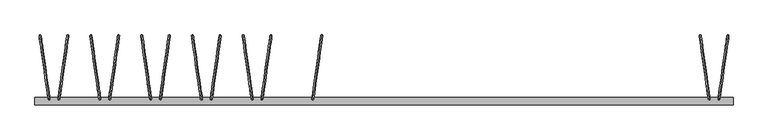
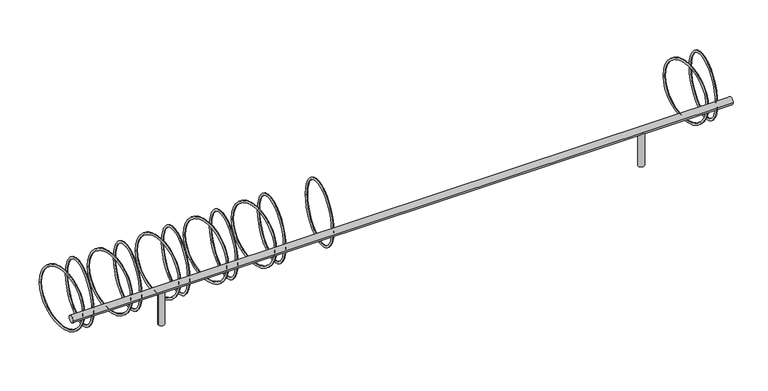
"""IFC4 building model written with IfcOpenShell, lengths in millimetres: geographic element geometry, NLRS_90_SI_WPB_fietsenrek staal_gen_bf : fietsenrek 5500mm 14 plaatsen."""

from ifc_helpers import new_model, si_unit, point, frame, frame_2d, origin, origin_with_axes, place, context, project, spatial, circle_curve, ellipse_curve, trimmed, segment, composite_curve, outline, extrude, source, transform, mapped, element, save
from ifc_brep_helpers import revolved_surface, advanced_brep


def geographic_element_aea35ce9(model_context):
    return source(origin(), model_context, "Body", "SolidModel", [
        advanced_brep(
        [(-560.5888305, 21.9255981, 304.7993564), (-562.7982034, 6.2050925, 304.7993564), (-489.8888952, 524.981777, 304.7993564), (-492.0982681, 509.2612714, 304.7993564)],
        [
            (0, 1, circle_curve(frame((-561.6935169, 14.0653453, 304.7993564), z_axis=(0.0, 0.0, 1.0), x_axis=(0.13917310096005764, 0.9902680687415715, 0.0)), 7.9375)),
            (1, 2, circle_curve(frame((-526.3435493, 265.5934347, 304.7993564), z_axis=(-0.9902680687415715, 0.1391731009600577, 0.0), x_axis=(0.1391731009600577, 0.9902680687415715, 0.0)), 261.9375)),
            (2, 3, circle_curve(frame((-490.9935817, 517.1215242, 304.7993564), z_axis=(0.0, 0.0, 1.0), x_axis=(-0.13917310096005775, -0.9902680687415715, 0.0)), 7.9375)),
            (3, 0, circle_curve(frame((-526.3435493, 265.5934347, 304.7993564), z_axis=(0.9902680687415715, -0.1391731009600577, 0.0), x_axis=(0.1391731009600577, 0.9902680687415715, 0.0)), 246.0625)),
            (1, 0, circle_curve(frame((-561.6935169, 14.0653453, 304.7993564), z_axis=(0.0, 0.0, 1.0), x_axis=(0.13917310096005764, 0.9902680687415715, 0.0)), 7.9375)),
            (3, 2, circle_curve(frame((-490.9935817, 517.1215242, 304.7993564), z_axis=(0.0, 0.0, 1.0), x_axis=(-0.13917310096005775, -0.9902680687415715, 0.0)), 7.9375)),
            (2, 1, circle_curve(frame((-526.3435493, 265.5934347, 304.7993564), z_axis=(-0.9902680687415715, 0.1391731009600577, 0.0), x_axis=(-0.1391731009600577, -0.9902680687415715, 0.0)), 261.9375)),
            (0, 3, circle_curve(frame((-526.3435493, 265.5934347, 304.7993564), z_axis=(0.9902680687415715, -0.1391731009600577, 0.0), x_axis=(-0.1391731009600577, -0.9902680687415715, 0.0)), 246.0625)),
        ],
        [
            revolved_surface(trimmed(ellipse_curve(frame((-490.9935817, 517.1215242, 304.7993564), z_axis=(0.0, 0.0, 1.0), x_axis=(-0.13917310096005775, -0.9902680687415715, 0.0)), 7.9375, 7.9375), [point((-489.8888952, 524.981777, 304.7993564))], [point((-492.0982681, 509.2612714, 304.7993564))], True, "CARTESIAN"), (-714.9896164, 292.1059105, 304.7993564), (-0.9902680687415715, 0.1391731009600577, 0.0)),
            revolved_surface(trimmed(ellipse_curve(frame((-490.9935817, 517.1215242, 304.7993564), z_axis=(0.0, 0.0, 1.0), x_axis=(-0.13917310096005775, -0.9902680687415715, 0.0)), 7.9375, 7.9375), [point((-492.0982681, 509.2612714, 304.7993564))], [point((-489.8888952, 524.981777, 304.7993564))], True, "CARTESIAN"), (-714.9896164, 292.1059105, 304.7993564), (-0.9902680687415715, 0.1391731009600577, 0.0)),
            revolved_surface(trimmed(ellipse_curve(frame((-561.6935169, 14.0653453, 304.7993564), z_axis=(0.0, 0.0, -1.0), x_axis=(0.1391731009600577, 0.9902680687415715, 0.0)), 7.9375, 7.9375), [point((-562.7982034, 6.2050925, 304.7993564))], [point((-560.5888305, 21.9255981, 304.7993564))], True, "CARTESIAN"), (-714.9896164, 292.1059105, 304.7993564), (-0.9902680687415715, 0.1391731009600577, 0.0)),
            revolved_surface(trimmed(ellipse_curve(frame((-561.6935169, 14.0653453, 304.7993564), z_axis=(0.0, 0.0, -1.0), x_axis=(0.1391731009600577, 0.9902680687415715, 0.0)), 7.9375, 7.9375), [point((-560.5888305, 21.9255981, 304.7993564))], [point((-562.7982034, 6.2050925, 304.7993564))], True, "CARTESIAN"), (-714.9896164, 292.1059105, 304.7993564), (-0.9902680687415715, 0.1391731009600577, 0.0)),
        ],
        [
            (0, [[1, 2, 3, 4]]),
            (1, [[5, -4, 6, -2]]),
            (2, [[-3, 7, -1, 8]]),
            (3, [[-6, -8, -5, -7]]),
        ],
    ),
        advanced_brep(
        [(-1039.4111695, 21.9255981, 304.7993564), (-1037.2017966, 6.2050925, 304.7993564), (-1110.1111048, 524.981777, 304.7993564), (-1107.9017319, 509.2612714, 304.7993564)],
        [
            (0, 1, circle_curve(frame((-1038.3064831, 14.0653453, 304.7993564), z_axis=(0.0, 0.0, 1.0), x_axis=(-0.1391731009600606, 0.990268068741571, 0.0)), 7.9375)),
            (1, 2, circle_curve(frame((-1073.6564507, 265.5934347, 304.7993564), z_axis=(-0.990268068741571, -0.13917310096006058, 0.0), x_axis=(-0.13917310096006058, 0.990268068741571, 0.0)), 261.9375)),
            (2, 3, circle_curve(frame((-1109.0064183, 517.1215242, 304.7993564), z_axis=(0.0, 0.0, 1.0), x_axis=(0.13917310096006055, -0.990268068741571, 0.0)), 7.9375)),
            (3, 0, circle_curve(frame((-1073.6564507, 265.5934347, 304.7993564), z_axis=(0.990268068741571, 0.13917310096006058, 0.0), x_axis=(-0.13917310096006058, 0.990268068741571, 0.0)), 246.0625)),
            (1, 0, circle_curve(frame((-1038.3064831, 14.0653453, 304.7993564), z_axis=(0.0, 0.0, 1.0), x_axis=(-0.1391731009600606, 0.990268068741571, 0.0)), 7.9375)),
            (3, 2, circle_curve(frame((-1109.0064183, 517.1215242, 304.7993564), z_axis=(0.0, 0.0, 1.0), x_axis=(0.13917310096006055, -0.990268068741571, 0.0)), 7.9375)),
            (2, 1, circle_curve(frame((-1073.6564507, 265.5934347, 304.7993564), z_axis=(-0.990268068741571, -0.13917310096006058, 0.0), x_axis=(0.13917310096006058, -0.990268068741571, 0.0)), 261.9375)),
            (0, 3, circle_curve(frame((-1073.6564507, 265.5934347, 304.7993564), z_axis=(0.990268068741571, 0.13917310096006058, 0.0), x_axis=(0.13917310096006058, -0.990268068741571, 0.0)), 246.0625)),
        ],
        [
            revolved_surface(trimmed(ellipse_curve(frame((-1109.0064183, 517.1215242, 304.7993564), z_axis=(0.0, 0.0, 1.0), x_axis=(0.13917310096006055, -0.990268068741571, 0.0)), 7.9375, 7.9375), [point((-1110.1111048, 524.981777, 304.7993564))], [point((-1107.9017319, 509.2612714, 304.7993564))], True, "CARTESIAN"), (-885.0103836, 292.1059105, 304.7993564), (-0.990268068741571, -0.13917310096006058, 0.0)),
            revolved_surface(trimmed(ellipse_curve(frame((-1109.0064183, 517.1215242, 304.7993564), z_axis=(0.0, 0.0, 1.0), x_axis=(0.13917310096006055, -0.990268068741571, 0.0)), 7.9375, 7.9375), [point((-1107.9017319, 509.2612714, 304.7993564))], [point((-1110.1111048, 524.981777, 304.7993564))], True, "CARTESIAN"), (-885.0103836, 292.1059105, 304.7993564), (-0.990268068741571, -0.13917310096006058, 0.0)),
            revolved_surface(trimmed(ellipse_curve(frame((-1038.3064831, 14.0653453, 304.7993564), z_axis=(0.0, 0.0, -1.0), x_axis=(-0.13917310096006055, 0.990268068741571, 0.0)), 7.9375, 7.9375), [point((-1037.2017966, 6.2050925, 304.7993564))], [point((-1039.4111695, 21.9255981, 304.7993564))], True, "CARTESIAN"), (-885.0103836, 292.1059105, 304.7993564), (-0.990268068741571, -0.13917310096006058, 0.0)),
            revolved_surface(trimmed(ellipse_curve(frame((-1038.3064831, 14.0653453, 304.7993564), z_axis=(0.0, 0.0, -1.0), x_axis=(-0.13917310096006055, 0.990268068741571, 0.0)), 7.9375, 7.9375), [point((-1039.4111695, 21.9255981, 304.7993564))], [point((-1037.2017966, 6.2050925, 304.7993564))], True, "CARTESIAN"), (-885.0103836, 292.1059105, 304.7993564), (-0.990268068741571, -0.13917310096006058, 0.0)),
        ],
        [
            (0, [[1, 2, 3, 4]]),
            (1, [[5, -4, 6, -2]]),
            (2, [[-3, 7, -1, 8]]),
            (3, [[-6, -8, -5, -7]]),
        ],
    ),
        advanced_brep(
        [(-960.5888305, 21.9255981, 304.7993564), (-962.7982034, 6.2050925, 304.7993564), (-889.8888952, 524.981777, 304.7993564), (-892.0982681, 509.2612714, 304.7993564)],
        [
            (0, 1, circle_curve(frame((-961.6935169, 14.0653453, 304.7993564), z_axis=(0.0, 0.0, 1.0), x_axis=(0.13917310096005764, 0.9902680687415715, 0.0)), 7.9375)),
            (1, 2, circle_curve(frame((-926.3435493, 265.5934347, 304.7993564), z_axis=(-0.9902680687415715, 0.1391731009600577, 0.0), x_axis=(0.1391731009600577, 0.9902680687415715, 0.0)), 261.9375)),
            (2, 3, circle_curve(frame((-890.9935817, 517.1215242, 304.7993564), z_axis=(0.0, 0.0, 1.0), x_axis=(-0.13917310096005775, -0.9902680687415715, 0.0)), 7.9375)),
            (3, 0, circle_curve(frame((-926.3435493, 265.5934347, 304.7993564), z_axis=(0.9902680687415715, -0.1391731009600577, 0.0), x_axis=(0.1391731009600577, 0.9902680687415715, 0.0)), 246.0625)),
            (1, 0, circle_curve(frame((-961.6935169, 14.0653453, 304.7993564), z_axis=(0.0, 0.0, 1.0), x_axis=(0.13917310096005764, 0.9902680687415715, 0.0)), 7.9375)),
            (3, 2, circle_curve(frame((-890.9935817, 517.1215242, 304.7993564), z_axis=(0.0, 0.0, 1.0), x_axis=(-0.13917310096005775, -0.9902680687415715, 0.0)), 7.9375)),
            (2, 1, circle_curve(frame((-926.3435493, 265.5934347, 304.7993564), z_axis=(-0.9902680687415715, 0.1391731009600577, 0.0), x_axis=(-0.1391731009600577, -0.9902680687415715, 0.0)), 261.9375)),
            (0, 3, circle_curve(frame((-926.3435493, 265.5934347, 304.7993564), z_axis=(0.9902680687415715, -0.1391731009600577, 0.0), x_axis=(-0.1391731009600577, -0.9902680687415715, 0.0)), 246.0625)),
        ],
        [
            revolved_surface(trimmed(ellipse_curve(frame((-890.9935817, 517.1215242, 304.7993564), z_axis=(0.0, 0.0, 1.0), x_axis=(-0.13917310096005775, -0.9902680687415715, 0.0)), 7.9375, 7.9375), [point((-889.8888952, 524.981777, 304.7993564))], [point((-892.0982681, 509.2612714, 304.7993564))], True, "CARTESIAN"), (-1114.9896164, 292.1059105, 304.7993564), (-0.9902680687415715, 0.1391731009600577, 0.0)),
            revolved_surface(trimmed(ellipse_curve(frame((-890.9935817, 517.1215242, 304.7993564), z_axis=(0.0, 0.0, 1.0), x_axis=(-0.13917310096005775, -0.9902680687415715, 0.0)), 7.9375, 7.9375), [point((-892.0982681, 509.2612714, 304.7993564))], [point((-889.8888952, 524.981777, 304.7993564))], True, "CARTESIAN"), (-1114.9896164, 292.1059105, 304.7993564), (-0.9902680687415715, 0.1391731009600577, 0.0)),
            revolved_surface(trimmed(ellipse_curve(frame((-961.6935169, 14.0653453, 304.7993564), z_axis=(0.0, 0.0, -1.0), x_axis=(0.1391731009600577, 0.9902680687415715, 0.0)), 7.9375, 7.9375), [point((-962.7982034, 6.2050925, 304.7993564))], [point((-960.5888305, 21.9255981, 304.7993564))], True, "CARTESIAN"), (-1114.9896164, 292.1059105, 304.7993564), (-0.9902680687415715, 0.1391731009600577, 0.0)),
            revolved_surface(trimmed(ellipse_curve(frame((-961.6935169, 14.0653453, 304.7993564), z_axis=(0.0, 0.0, -1.0), x_axis=(0.1391731009600577, 0.9902680687415715, 0.0)), 7.9375, 7.9375), [point((-960.5888305, 21.9255981, 304.7993564))], [point((-962.7982034, 6.2050925, 304.7993564))], True, "CARTESIAN"), (-1114.9896164, 292.1059105, 304.7993564), (-0.9902680687415715, 0.1391731009600577, 0.0)),
        ],
        [
            (0, [[1, 2, 3, 4]]),
            (1, [[5, -4, 6, -2]]),
            (2, [[-3, 7, -1, 8]]),
            (3, [[-6, -8, -5, -7]]),
        ],
    ),
        advanced_brep(
        [(-1439.4111695, 21.9255981, 304.7993564), (-1437.2017966, 6.2050925, 304.7993564), (-1510.1111048, 524.981777, 304.7993564), (-1507.9017319, 509.2612714, 304.7993564)],
        [
            (0, 1, circle_curve(frame((-1438.3064831, 14.0653453, 304.7993564), z_axis=(0.0, 0.0, 1.0), x_axis=(-0.1391731009600606, 0.990268068741571, 0.0)), 7.9375)),
            (1, 2, circle_curve(frame((-1473.6564507, 265.5934347, 304.7993564), z_axis=(-0.990268068741571, -0.13917310096006058, 0.0), x_axis=(-0.13917310096006058, 0.990268068741571, 0.0)), 261.9375)),
            (2, 3, circle_curve(frame((-1509.0064183, 517.1215242, 304.7993564), z_axis=(0.0, 0.0, 1.0), x_axis=(0.13917310096006055, -0.990268068741571, 0.0)), 7.9375)),
            (3, 0, circle_curve(frame((-1473.6564507, 265.5934347, 304.7993564), z_axis=(0.990268068741571, 0.13917310096006058, 0.0), x_axis=(-0.13917310096006058, 0.990268068741571, 0.0)), 246.0625)),
            (1, 0, circle_curve(frame((-1438.3064831, 14.0653453, 304.7993564), z_axis=(0.0, 0.0, 1.0), x_axis=(-0.1391731009600606, 0.990268068741571, 0.0)), 7.9375)),
            (3, 2, circle_curve(frame((-1509.0064183, 517.1215242, 304.7993564), z_axis=(0.0, 0.0, 1.0), x_axis=(0.13917310096006055, -0.990268068741571, 0.0)), 7.9375)),
            (2, 1, circle_curve(frame((-1473.6564507, 265.5934347, 304.7993564), z_axis=(-0.990268068741571, -0.13917310096006058, 0.0), x_axis=(0.13917310096006058, -0.990268068741571, 0.0)), 261.9375)),
            (0, 3, circle_curve(frame((-1473.6564507, 265.5934347, 304.7993564), z_axis=(0.990268068741571, 0.13917310096006058, 0.0), x_axis=(0.13917310096006058, -0.990268068741571, 0.0)), 246.0625)),
        ],
        [
            revolved_surface(trimmed(ellipse_curve(frame((-1509.0064183, 517.1215242, 304.7993564), z_axis=(0.0, 0.0, 1.0), x_axis=(0.13917310096006055, -0.990268068741571, 0.0)), 7.9375, 7.9375), [point((-1510.1111048, 524.981777, 304.7993564))], [point((-1507.9017319, 509.2612714, 304.7993564))], True, "CARTESIAN"), (-1285.0103836, 292.1059105, 304.7993564), (-0.990268068741571, -0.13917310096006058, 0.0)),
            revolved_surface(trimmed(ellipse_curve(frame((-1509.0064183, 517.1215242, 304.7993564), z_axis=(0.0, 0.0, 1.0), x_axis=(0.13917310096006055, -0.990268068741571, 0.0)), 7.9375, 7.9375), [point((-1507.9017319, 509.2612714, 304.7993564))], [point((-1510.1111048, 524.981777, 304.7993564))], True, "CARTESIAN"), (-1285.0103836, 292.1059105, 304.7993564), (-0.990268068741571, -0.13917310096006058, 0.0)),
            revolved_surface(trimmed(ellipse_curve(frame((-1438.3064831, 14.0653453, 304.7993564), z_axis=(0.0, 0.0, -1.0), x_axis=(-0.13917310096006055, 0.990268068741571, 0.0)), 7.9375, 7.9375), [point((-1437.2017966, 6.2050925, 304.7993564))], [point((-1439.4111695, 21.9255981, 304.7993564))], True, "CARTESIAN"), (-1285.0103836, 292.1059105, 304.7993564), (-0.990268068741571, -0.13917310096006058, 0.0)),
            revolved_surface(trimmed(ellipse_curve(frame((-1438.3064831, 14.0653453, 304.7993564), z_axis=(0.0, 0.0, -1.0), x_axis=(-0.13917310096006055, 0.990268068741571, 0.0)), 7.9375, 7.9375), [point((-1439.4111695, 21.9255981, 304.7993564))], [point((-1437.2017966, 6.2050925, 304.7993564))], True, "CARTESIAN"), (-1285.0103836, 292.1059105, 304.7993564), (-0.990268068741571, -0.13917310096006058, 0.0)),
        ],
        [
            (0, [[1, 2, 3, 4]]),
            (1, [[5, -4, 6, -2]]),
            (2, [[-3, 7, -1, 8]]),
            (3, [[-6, -8, -5, -7]]),
        ],
    ),
        advanced_brep(
        [(-1360.5888305, 21.9255981, 304.7993564), (-1362.7982034, 6.2050925, 304.7993564), (-1289.8888952, 524.981777, 304.7993564), (-1292.0982681, 509.2612714, 304.7993564)],
        [
            (0, 1, circle_curve(frame((-1361.6935169, 14.0653453, 304.7993564), z_axis=(0.0, 0.0, 1.0), x_axis=(0.13917310096005764, 0.9902680687415715, 0.0)), 7.9375)),
            (1, 2, circle_curve(frame((-1326.3435493, 265.5934347, 304.7993564), z_axis=(-0.9902680687415715, 0.1391731009600577, 0.0), x_axis=(0.1391731009600577, 0.9902680687415715, 0.0)), 261.9375)),
            (2, 3, circle_curve(frame((-1290.9935817, 517.1215242, 304.7993564), z_axis=(0.0, 0.0, 1.0), x_axis=(-0.13917310096005775, -0.9902680687415715, 0.0)), 7.9375)),
            (3, 0, circle_curve(frame((-1326.3435493, 265.5934347, 304.7993564), z_axis=(0.9902680687415715, -0.1391731009600577, 0.0), x_axis=(0.1391731009600577, 0.9902680687415715, 0.0)), 246.0625)),
            (1, 0, circle_curve(frame((-1361.6935169, 14.0653453, 304.7993564), z_axis=(0.0, 0.0, 1.0), x_axis=(0.13917310096005764, 0.9902680687415715, 0.0)), 7.9375)),
            (3, 2, circle_curve(frame((-1290.9935817, 517.1215242, 304.7993564), z_axis=(0.0, 0.0, 1.0), x_axis=(-0.13917310096005775, -0.9902680687415715, 0.0)), 7.9375)),
            (2, 1, circle_curve(frame((-1326.3435493, 265.5934347, 304.7993564), z_axis=(-0.9902680687415715, 0.1391731009600577, 0.0), x_axis=(-0.1391731009600577, -0.9902680687415715, 0.0)), 261.9375)),
            (0, 3, circle_curve(frame((-1326.3435493, 265.5934347, 304.7993564), z_axis=(0.9902680687415715, -0.1391731009600577, 0.0), x_axis=(-0.1391731009600577, -0.9902680687415715, 0.0)), 246.0625)),
        ],
        [
            revolved_surface(trimmed(ellipse_curve(frame((-1290.9935817, 517.1215242, 304.7993564), z_axis=(0.0, 0.0, 1.0), x_axis=(-0.13917310096005775, -0.9902680687415715, 0.0)), 7.9375, 7.9375), [point((-1289.8888952, 524.981777, 304.7993564))], [point((-1292.0982681, 509.2612714, 304.7993564))], True, "CARTESIAN"), (-1514.9896164, 292.1059105, 304.7993564), (-0.9902680687415715, 0.1391731009600577, 0.0)),
            revolved_surface(trimmed(ellipse_curve(frame((-1290.9935817, 517.1215242, 304.7993564), z_axis=(0.0, 0.0, 1.0), x_axis=(-0.13917310096005775, -0.9902680687415715, 0.0)), 7.9375, 7.9375), [point((-1292.0982681, 509.2612714, 304.7993564))], [point((-1289.8888952, 524.981777, 304.7993564))], True, "CARTESIAN"), (-1514.9896164, 292.1059105, 304.7993564), (-0.9902680687415715, 0.1391731009600577, 0.0)),
            revolved_surface(trimmed(ellipse_curve(frame((-1361.6935169, 14.0653453, 304.7993564), z_axis=(0.0, 0.0, -1.0), x_axis=(0.1391731009600577, 0.9902680687415715, 0.0)), 7.9375, 7.9375), [point((-1362.7982034, 6.2050925, 304.7993564))], [point((-1360.5888305, 21.9255981, 304.7993564))], True, "CARTESIAN"), (-1514.9896164, 292.1059105, 304.7993564), (-0.9902680687415715, 0.1391731009600577, 0.0)),
            revolved_surface(trimmed(ellipse_curve(frame((-1361.6935169, 14.0653453, 304.7993564), z_axis=(0.0, 0.0, -1.0), x_axis=(0.1391731009600577, 0.9902680687415715, 0.0)), 7.9375, 7.9375), [point((-1360.5888305, 21.9255981, 304.7993564))], [point((-1362.7982034, 6.2050925, 304.7993564))], True, "CARTESIAN"), (-1514.9896164, 292.1059105, 304.7993564), (-0.9902680687415715, 0.1391731009600577, 0.0)),
        ],
        [
            (0, [[1, 2, 3, 4]]),
            (1, [[5, -4, 6, -2]]),
            (2, [[-3, 7, -1, 8]]),
            (3, [[-6, -8, -5, -7]]),
        ],
    ),
        advanced_brep(
        [(-1839.4111695, 21.9255981, 304.7993564), (-1837.2017966, 6.2050925, 304.7993564), (-1910.1111048, 524.981777, 304.7993564), (-1907.9017319, 509.2612714, 304.7993564)],
        [
            (0, 1, circle_curve(frame((-1838.3064831, 14.0653453, 304.7993564), z_axis=(0.0, 0.0, 1.0), x_axis=(-0.1391731009600606, 0.990268068741571, 0.0)), 7.9375)),
            (1, 2, circle_curve(frame((-1873.6564507, 265.5934347, 304.7993564), z_axis=(-0.990268068741571, -0.13917310096006058, 0.0), x_axis=(-0.13917310096006058, 0.990268068741571, 0.0)), 261.9375)),
            (2, 3, circle_curve(frame((-1909.0064183, 517.1215242, 304.7993564), z_axis=(0.0, 0.0, 1.0), x_axis=(0.13917310096006055, -0.990268068741571, 0.0)), 7.9375)),
            (3, 0, circle_curve(frame((-1873.6564507, 265.5934347, 304.7993564), z_axis=(0.990268068741571, 0.13917310096006058, 0.0), x_axis=(-0.13917310096006058, 0.990268068741571, 0.0)), 246.0625)),
            (1, 0, circle_curve(frame((-1838.3064831, 14.0653453, 304.7993564), z_axis=(0.0, 0.0, 1.0), x_axis=(-0.1391731009600606, 0.990268068741571, 0.0)), 7.9375)),
            (3, 2, circle_curve(frame((-1909.0064183, 517.1215242, 304.7993564), z_axis=(0.0, 0.0, 1.0), x_axis=(0.13917310096006055, -0.990268068741571, 0.0)), 7.9375)),
            (2, 1, circle_curve(frame((-1873.6564507, 265.5934347, 304.7993564), z_axis=(-0.990268068741571, -0.13917310096006058, 0.0), x_axis=(0.13917310096006058, -0.990268068741571, 0.0)), 261.9375)),
            (0, 3, circle_curve(frame((-1873.6564507, 265.5934347, 304.7993564), z_axis=(0.990268068741571, 0.13917310096006058, 0.0), x_axis=(0.13917310096006058, -0.990268068741571, 0.0)), 246.0625)),
        ],
        [
            revolved_surface(trimmed(ellipse_curve(frame((-1909.0064183, 517.1215242, 304.7993564), z_axis=(0.0, 0.0, 1.0), x_axis=(0.13917310096006055, -0.990268068741571, 0.0)), 7.9375, 7.9375), [point((-1910.1111048, 524.981777, 304.7993564))], [point((-1907.9017319, 509.2612714, 304.7993564))], True, "CARTESIAN"), (-1685.0103836, 292.1059105, 304.7993564), (-0.990268068741571, -0.13917310096006058, 0.0)),
            revolved_surface(trimmed(ellipse_curve(frame((-1909.0064183, 517.1215242, 304.7993564), z_axis=(0.0, 0.0, 1.0), x_axis=(0.13917310096006055, -0.990268068741571, 0.0)), 7.9375, 7.9375), [point((-1907.9017319, 509.2612714, 304.7993564))], [point((-1910.1111048, 524.981777, 304.7993564))], True, "CARTESIAN"), (-1685.0103836, 292.1059105, 304.7993564), (-0.990268068741571, -0.13917310096006058, 0.0)),
            revolved_surface(trimmed(ellipse_curve(frame((-1838.3064831, 14.0653453, 304.7993564), z_axis=(0.0, 0.0, -1.0), x_axis=(-0.13917310096006055, 0.990268068741571, 0.0)), 7.9375, 7.9375), [point((-1837.2017966, 6.2050925, 304.7993564))], [point((-1839.4111695, 21.9255981, 304.7993564))], True, "CARTESIAN"), (-1685.0103836, 292.1059105, 304.7993564), (-0.990268068741571, -0.13917310096006058, 0.0)),
            revolved_surface(trimmed(ellipse_curve(frame((-1838.3064831, 14.0653453, 304.7993564), z_axis=(0.0, 0.0, -1.0), x_axis=(-0.13917310096006055, 0.990268068741571, 0.0)), 7.9375, 7.9375), [point((-1839.4111695, 21.9255981, 304.7993564))], [point((-1837.2017966, 6.2050925, 304.7993564))], True, "CARTESIAN"), (-1685.0103836, 292.1059105, 304.7993564), (-0.990268068741571, -0.13917310096006058, 0.0)),
        ],
        [
            (0, [[1, 2, 3, 4]]),
            (1, [[5, -4, 6, -2]]),
            (2, [[-3, 7, -1, 8]]),
            (3, [[-6, -8, -5, -7]]),
        ],
    ),
        advanced_brep(
        [(-1760.5888305, 21.9255981, 304.7993564), (-1762.7982034, 6.2050925, 304.7993564), (-1689.8888952, 524.981777, 304.7993564), (-1692.0982681, 509.2612714, 304.7993564)],
        [
            (0, 1, circle_curve(frame((-1761.6935169, 14.0653453, 304.7993564), z_axis=(0.0, 0.0, 1.0), x_axis=(0.13917310096005764, 0.9902680687415715, 0.0)), 7.9375)),
            (1, 2, circle_curve(frame((-1726.3435493, 265.5934347, 304.7993564), z_axis=(-0.9902680687415715, 0.1391731009600577, 0.0), x_axis=(0.1391731009600577, 0.9902680687415715, 0.0)), 261.9375)),
            (2, 3, circle_curve(frame((-1690.9935817, 517.1215242, 304.7993564), z_axis=(0.0, 0.0, 1.0), x_axis=(-0.13917310096005775, -0.9902680687415715, 0.0)), 7.9375)),
            (3, 0, circle_curve(frame((-1726.3435493, 265.5934347, 304.7993564), z_axis=(0.9902680687415715, -0.1391731009600577, 0.0), x_axis=(0.1391731009600577, 0.9902680687415715, 0.0)), 246.0625)),
            (1, 0, circle_curve(frame((-1761.6935169, 14.0653453, 304.7993564), z_axis=(0.0, 0.0, 1.0), x_axis=(0.13917310096005764, 0.9902680687415715, 0.0)), 7.9375)),
            (3, 2, circle_curve(frame((-1690.9935817, 517.1215242, 304.7993564), z_axis=(0.0, 0.0, 1.0), x_axis=(-0.13917310096005775, -0.9902680687415715, 0.0)), 7.9375)),
            (2, 1, circle_curve(frame((-1726.3435493, 265.5934347, 304.7993564), z_axis=(-0.9902680687415715, 0.1391731009600577, 0.0), x_axis=(-0.1391731009600577, -0.9902680687415715, 0.0)), 261.9375)),
            (0, 3, circle_curve(frame((-1726.3435493, 265.5934347, 304.7993564), z_axis=(0.9902680687415715, -0.1391731009600577, 0.0), x_axis=(-0.1391731009600577, -0.9902680687415715, 0.0)), 246.0625)),
        ],
        [
            revolved_surface(trimmed(ellipse_curve(frame((-1690.9935817, 517.1215242, 304.7993564), z_axis=(0.0, 0.0, 1.0), x_axis=(-0.13917310096005775, -0.9902680687415715, 0.0)), 7.9375, 7.9375), [point((-1689.8888952, 524.981777, 304.7993564))], [point((-1692.0982681, 509.2612714, 304.7993564))], True, "CARTESIAN"), (-1914.9896164, 292.1059105, 304.7993564), (-0.9902680687415715, 0.1391731009600577, 0.0)),
            revolved_surface(trimmed(ellipse_curve(frame((-1690.9935817, 517.1215242, 304.7993564), z_axis=(0.0, 0.0, 1.0), x_axis=(-0.13917310096005775, -0.9902680687415715, 0.0)), 7.9375, 7.9375), [point((-1692.0982681, 509.2612714, 304.7993564))], [point((-1689.8888952, 524.981777, 304.7993564))], True, "CARTESIAN"), (-1914.9896164, 292.1059105, 304.7993564), (-0.9902680687415715, 0.1391731009600577, 0.0)),
            revolved_surface(trimmed(ellipse_curve(frame((-1761.6935169, 14.0653453, 304.7993564), z_axis=(0.0, 0.0, -1.0), x_axis=(0.1391731009600577, 0.9902680687415715, 0.0)), 7.9375, 7.9375), [point((-1762.7982034, 6.2050925, 304.7993564))], [point((-1760.5888305, 21.9255981, 304.7993564))], True, "CARTESIAN"), (-1914.9896164, 292.1059105, 304.7993564), (-0.9902680687415715, 0.1391731009600577, 0.0)),
            revolved_surface(trimmed(ellipse_curve(frame((-1761.6935169, 14.0653453, 304.7993564), z_axis=(0.0, 0.0, -1.0), x_axis=(0.1391731009600577, 0.9902680687415715, 0.0)), 7.9375, 7.9375), [point((-1760.5888305, 21.9255981, 304.7993564))], [point((-1762.7982034, 6.2050925, 304.7993564))], True, "CARTESIAN"), (-1914.9896164, 292.1059105, 304.7993564), (-0.9902680687415715, 0.1391731009600577, 0.0)),
        ],
        [
            (0, [[1, 2, 3, 4]]),
            (1, [[5, -4, 6, -2]]),
            (2, [[-3, 7, -1, 8]]),
            (3, [[-6, -8, -5, -7]]),
        ],
    ),
        advanced_brep(
        [(-2239.4111695, 21.9255981, 304.7993564), (-2237.2017966, 6.2050925, 304.7993564), (-2310.1111048, 524.981777, 304.7993564), (-2307.9017319, 509.2612714, 304.7993564)],
        [
            (0, 1, circle_curve(frame((-2238.3064831, 14.0653453, 304.7993564), z_axis=(0.0, 0.0, 1.0), x_axis=(-0.1391731009600606, 0.990268068741571, 0.0)), 7.9375)),
            (1, 2, circle_curve(frame((-2273.6564507, 265.5934347, 304.7993564), z_axis=(-0.990268068741571, -0.13917310096006058, 0.0), x_axis=(-0.13917310096006058, 0.990268068741571, 0.0)), 261.9375)),
            (2, 3, circle_curve(frame((-2309.0064183, 517.1215242, 304.7993564), z_axis=(0.0, 0.0, 1.0), x_axis=(0.13917310096006055, -0.990268068741571, 0.0)), 7.9375)),
            (3, 0, circle_curve(frame((-2273.6564507, 265.5934347, 304.7993564), z_axis=(0.990268068741571, 0.13917310096006058, 0.0), x_axis=(-0.13917310096006058, 0.990268068741571, 0.0)), 246.0625)),
            (1, 0, circle_curve(frame((-2238.3064831, 14.0653453, 304.7993564), z_axis=(0.0, 0.0, 1.0), x_axis=(-0.1391731009600606, 0.990268068741571, 0.0)), 7.9375)),
            (3, 2, circle_curve(frame((-2309.0064183, 517.1215242, 304.7993564), z_axis=(0.0, 0.0, 1.0), x_axis=(0.13917310096006055, -0.990268068741571, 0.0)), 7.9375)),
            (2, 1, circle_curve(frame((-2273.6564507, 265.5934347, 304.7993564), z_axis=(-0.990268068741571, -0.13917310096006058, 0.0), x_axis=(0.13917310096006058, -0.990268068741571, 0.0)), 261.9375)),
            (0, 3, circle_curve(frame((-2273.6564507, 265.5934347, 304.7993564), z_axis=(0.990268068741571, 0.13917310096006058, 0.0), x_axis=(0.13917310096006058, -0.990268068741571, 0.0)), 246.0625)),
        ],
        [
            revolved_surface(trimmed(ellipse_curve(frame((-2309.0064183, 517.1215242, 304.7993564), z_axis=(0.0, 0.0, 1.0), x_axis=(0.13917310096006055, -0.990268068741571, 0.0)), 7.9375, 7.9375), [point((-2310.1111048, 524.981777, 304.7993564))], [point((-2307.9017319, 509.2612714, 304.7993564))], True, "CARTESIAN"), (-2085.0103836, 292.1059105, 304.7993564), (-0.990268068741571, -0.13917310096006058, 0.0)),
            revolved_surface(trimmed(ellipse_curve(frame((-2309.0064183, 517.1215242, 304.7993564), z_axis=(0.0, 0.0, 1.0), x_axis=(0.13917310096006055, -0.990268068741571, 0.0)), 7.9375, 7.9375), [point((-2307.9017319, 509.2612714, 304.7993564))], [point((-2310.1111048, 524.981777, 304.7993564))], True, "CARTESIAN"), (-2085.0103836, 292.1059105, 304.7993564), (-0.990268068741571, -0.13917310096006058, 0.0)),
            revolved_surface(trimmed(ellipse_curve(frame((-2238.3064831, 14.0653453, 304.7993564), z_axis=(0.0, 0.0, -1.0), x_axis=(-0.13917310096006055, 0.990268068741571, 0.0)), 7.9375, 7.9375), [point((-2237.2017966, 6.2050925, 304.7993564))], [point((-2239.4111695, 21.9255981, 304.7993564))], True, "CARTESIAN"), (-2085.0103836, 292.1059105, 304.7993564), (-0.990268068741571, -0.13917310096006058, 0.0)),
            revolved_surface(trimmed(ellipse_curve(frame((-2238.3064831, 14.0653453, 304.7993564), z_axis=(0.0, 0.0, -1.0), x_axis=(-0.13917310096006055, 0.990268068741571, 0.0)), 7.9375, 7.9375), [point((-2239.4111695, 21.9255981, 304.7993564))], [point((-2237.2017966, 6.2050925, 304.7993564))], True, "CARTESIAN"), (-2085.0103836, 292.1059105, 304.7993564), (-0.990268068741571, -0.13917310096006058, 0.0)),
        ],
        [
            (0, [[1, 2, 3, 4]]),
            (1, [[5, -4, 6, -2]]),
            (2, [[-3, 7, -1, 8]]),
            (3, [[-6, -8, -5, -7]]),
        ],
    ),
        advanced_brep(
        [(-2160.5888305, 21.9255981, 304.7993564), (-2162.7982034, 6.2050925, 304.7993564), (-2089.8888952, 524.981777, 304.7993564), (-2092.0982681, 509.2612714, 304.7993564)],
        [
            (0, 1, circle_curve(frame((-2161.6935169, 14.0653453, 304.7993564), z_axis=(0.0, 0.0, 1.0), x_axis=(0.13917310096005764, 0.9902680687415715, 0.0)), 7.9375)),
            (1, 2, circle_curve(frame((-2126.3435493, 265.5934347, 304.7993564), z_axis=(-0.9902680687415715, 0.1391731009600577, 0.0), x_axis=(0.1391731009600577, 0.9902680687415715, 0.0)), 261.9375)),
            (2, 3, circle_curve(frame((-2090.9935817, 517.1215242, 304.7993564), z_axis=(0.0, 0.0, 1.0), x_axis=(-0.13917310096005775, -0.9902680687415715, 0.0)), 7.9375)),
            (3, 0, circle_curve(frame((-2126.3435493, 265.5934347, 304.7993564), z_axis=(0.9902680687415715, -0.1391731009600577, 0.0), x_axis=(0.1391731009600577, 0.9902680687415715, 0.0)), 246.0625)),
            (1, 0, circle_curve(frame((-2161.6935169, 14.0653453, 304.7993564), z_axis=(0.0, 0.0, 1.0), x_axis=(0.13917310096005764, 0.9902680687415715, 0.0)), 7.9375)),
            (3, 2, circle_curve(frame((-2090.9935817, 517.1215242, 304.7993564), z_axis=(0.0, 0.0, 1.0), x_axis=(-0.13917310096005775, -0.9902680687415715, 0.0)), 7.9375)),
            (2, 1, circle_curve(frame((-2126.3435493, 265.5934347, 304.7993564), z_axis=(-0.9902680687415715, 0.1391731009600577, 0.0), x_axis=(-0.1391731009600577, -0.9902680687415715, 0.0)), 261.9375)),
            (0, 3, circle_curve(frame((-2126.3435493, 265.5934347, 304.7993564), z_axis=(0.9902680687415715, -0.1391731009600577, 0.0), x_axis=(-0.1391731009600577, -0.9902680687415715, 0.0)), 246.0625)),
        ],
        [
            revolved_surface(trimmed(ellipse_curve(frame((-2090.9935817, 517.1215242, 304.7993564), z_axis=(0.0, 0.0, 1.0), x_axis=(-0.13917310096005775, -0.9902680687415715, 0.0)), 7.9375, 7.9375), [point((-2089.8888952, 524.981777, 304.7993564))], [point((-2092.0982681, 509.2612714, 304.7993564))], True, "CARTESIAN"), (-2314.9896164, 292.1059105, 304.7993564), (-0.9902680687415715, 0.1391731009600577, 0.0)),
            revolved_surface(trimmed(ellipse_curve(frame((-2090.9935817, 517.1215242, 304.7993564), z_axis=(0.0, 0.0, 1.0), x_axis=(-0.13917310096005775, -0.9902680687415715, 0.0)), 7.9375, 7.9375), [point((-2092.0982681, 509.2612714, 304.7993564))], [point((-2089.8888952, 524.981777, 304.7993564))], True, "CARTESIAN"), (-2314.9896164, 292.1059105, 304.7993564), (-0.9902680687415715, 0.1391731009600577, 0.0)),
            revolved_surface(trimmed(ellipse_curve(frame((-2161.6935169, 14.0653453, 304.7993564), z_axis=(0.0, 0.0, -1.0), x_axis=(0.1391731009600577, 0.9902680687415715, 0.0)), 7.9375, 7.9375), [point((-2162.7982034, 6.2050925, 304.7993564))], [point((-2160.5888305, 21.9255981, 304.7993564))], True, "CARTESIAN"), (-2314.9896164, 292.1059105, 304.7993564), (-0.9902680687415715, 0.1391731009600577, 0.0)),
            revolved_surface(trimmed(ellipse_curve(frame((-2161.6935169, 14.0653453, 304.7993564), z_axis=(0.0, 0.0, -1.0), x_axis=(0.1391731009600577, 0.9902680687415715, 0.0)), 7.9375, 7.9375), [point((-2160.5888305, 21.9255981, 304.7993564))], [point((-2162.7982034, 6.2050925, 304.7993564))], True, "CARTESIAN"), (-2314.9896164, 292.1059105, 304.7993564), (-0.9902680687415715, 0.1391731009600577, 0.0)),
        ],
        [
            (0, [[1, 2, 3, 4]]),
            (1, [[5, -4, 6, -2]]),
            (2, [[-3, 7, -1, 8]]),
            (3, [[-6, -8, -5, -7]]),
        ],
    ),
        advanced_brep(
        [(2560.5888305, 21.9255981, 304.7993564), (2562.7982034, 6.2050925, 304.7993564), (2489.8888952, 524.981777, 304.7993564), (2492.0982681, 509.2612714, 304.7993564)],
        [
            (0, 1, circle_curve(frame((2561.6935169, 14.0653453, 304.7993564), z_axis=(0.0, 0.0, 1.0), x_axis=(-0.1391731009600606, 0.990268068741571, 0.0)), 7.9375)),
            (1, 2, circle_curve(frame((2526.3435493, 265.5934347, 304.7993564), z_axis=(-0.990268068741571, -0.13917310096006058, 0.0), x_axis=(-0.13917310096006058, 0.990268068741571, 0.0)), 261.9375)),
            (2, 3, circle_curve(frame((2490.9935817, 517.1215242, 304.7993564), z_axis=(0.0, 0.0, 1.0), x_axis=(0.13917310096006055, -0.990268068741571, 0.0)), 7.9375)),
            (3, 0, circle_curve(frame((2526.3435493, 265.5934347, 304.7993564), z_axis=(0.990268068741571, 0.13917310096006058, 0.0), x_axis=(-0.13917310096006058, 0.990268068741571, 0.0)), 246.0625)),
            (1, 0, circle_curve(frame((2561.6935169, 14.0653453, 304.7993564), z_axis=(0.0, 0.0, 1.0), x_axis=(-0.1391731009600606, 0.990268068741571, 0.0)), 7.9375)),
            (3, 2, circle_curve(frame((2490.9935817, 517.1215242, 304.7993564), z_axis=(0.0, 0.0, 1.0), x_axis=(0.13917310096006055, -0.990268068741571, 0.0)), 7.9375)),
            (2, 1, circle_curve(frame((2526.3435493, 265.5934347, 304.7993564), z_axis=(-0.990268068741571, -0.13917310096006058, 0.0), x_axis=(0.13917310096006058, -0.990268068741571, 0.0)), 261.9375)),
            (0, 3, circle_curve(frame((2526.3435493, 265.5934347, 304.7993564), z_axis=(0.990268068741571, 0.13917310096006058, 0.0), x_axis=(0.13917310096006058, -0.990268068741571, 0.0)), 246.0625)),
        ],
        [
            revolved_surface(trimmed(ellipse_curve(frame((2490.9935817, 517.1215242, 304.7993564), z_axis=(0.0, 0.0, 1.0), x_axis=(0.13917310096006055, -0.990268068741571, 0.0)), 7.9375, 7.9375), [point((2489.8888952, 524.981777, 304.7993564))], [point((2492.0982681, 509.2612714, 304.7993564))], True, "CARTESIAN"), (2714.9896164, 292.1059105, 304.7993564), (-0.990268068741571, -0.13917310096006058, 0.0)),
            revolved_surface(trimmed(ellipse_curve(frame((2490.9935817, 517.1215242, 304.7993564), z_axis=(0.0, 0.0, 1.0), x_axis=(0.13917310096006055, -0.990268068741571, 0.0)), 7.9375, 7.9375), [point((2492.0982681, 509.2612714, 304.7993564))], [point((2489.8888952, 524.981777, 304.7993564))], True, "CARTESIAN"), (2714.9896164, 292.1059105, 304.7993564), (-0.990268068741571, -0.13917310096006058, 0.0)),
            revolved_surface(trimmed(ellipse_curve(frame((2561.6935169, 14.0653453, 304.7993564), z_axis=(0.0, 0.0, -1.0), x_axis=(-0.13917310096006055, 0.990268068741571, 0.0)), 7.9375, 7.9375), [point((2562.7982034, 6.2050925, 304.7993564))], [point((2560.5888305, 21.9255981, 304.7993564))], True, "CARTESIAN"), (2714.9896164, 292.1059105, 304.7993564), (-0.990268068741571, -0.13917310096006058, 0.0)),
            revolved_surface(trimmed(ellipse_curve(frame((2561.6935169, 14.0653453, 304.7993564), z_axis=(0.0, 0.0, -1.0), x_axis=(-0.13917310096006055, 0.990268068741571, 0.0)), 7.9375, 7.9375), [point((2560.5888305, 21.9255981, 304.7993564))], [point((2562.7982034, 6.2050925, 304.7993564))], True, "CARTESIAN"), (2714.9896164, 292.1059105, 304.7993564), (-0.990268068741571, -0.13917310096006058, 0.0)),
        ],
        [
            (0, [[1, 2, 3, 4]]),
            (1, [[5, -4, 6, -2]]),
            (2, [[-3, 7, -1, 8]]),
            (3, [[-6, -8, -5, -7]]),
        ],
    ),
        advanced_brep(
        [(2639.4111695, 21.9255981, 304.7993564), (2637.2017966, 6.2050925, 304.7993564), (2710.1111048, 524.981777, 304.7993564), (2707.9017319, 509.2612714, 304.7993564)],
        [
            (0, 1, circle_curve(frame((2638.3064831, 14.0653453, 304.7993564), z_axis=(0.0, 0.0, 1.0), x_axis=(0.13917310096005764, 0.9902680687415715, 0.0)), 7.9375)),
            (1, 2, circle_curve(frame((2673.6564507, 265.5934347, 304.7993564), z_axis=(-0.9902680687415715, 0.1391731009600577, 0.0), x_axis=(0.1391731009600577, 0.9902680687415715, 0.0)), 261.9375)),
            (2, 3, circle_curve(frame((2709.0064183, 517.1215242, 304.7993564), z_axis=(0.0, 0.0, 1.0), x_axis=(-0.13917310096005775, -0.9902680687415715, 0.0)), 7.9375)),
            (3, 0, circle_curve(frame((2673.6564507, 265.5934347, 304.7993564), z_axis=(0.9902680687415715, -0.1391731009600577, 0.0), x_axis=(0.1391731009600577, 0.9902680687415715, 0.0)), 246.0625)),
            (1, 0, circle_curve(frame((2638.3064831, 14.0653453, 304.7993564), z_axis=(0.0, 0.0, 1.0), x_axis=(0.13917310096005764, 0.9902680687415715, 0.0)), 7.9375)),
            (3, 2, circle_curve(frame((2709.0064183, 517.1215242, 304.7993564), z_axis=(0.0, 0.0, 1.0), x_axis=(-0.13917310096005775, -0.9902680687415715, 0.0)), 7.9375)),
            (2, 1, circle_curve(frame((2673.6564507, 265.5934347, 304.7993564), z_axis=(-0.9902680687415715, 0.1391731009600577, 0.0), x_axis=(-0.1391731009600577, -0.9902680687415715, 0.0)), 261.9375)),
            (0, 3, circle_curve(frame((2673.6564507, 265.5934347, 304.7993564), z_axis=(0.9902680687415715, -0.1391731009600577, 0.0), x_axis=(-0.1391731009600577, -0.9902680687415715, 0.0)), 246.0625)),
        ],
        [
            revolved_surface(trimmed(ellipse_curve(frame((2709.0064183, 517.1215242, 304.7993564), z_axis=(0.0, 0.0, 1.0), x_axis=(-0.13917310096005775, -0.9902680687415715, 0.0)), 7.9375, 7.9375), [point((2710.1111048, 524.981777, 304.7993564))], [point((2707.9017319, 509.2612714, 304.7993564))], True, "CARTESIAN"), (2485.0103836, 292.1059105, 304.7993564), (-0.9902680687415715, 0.1391731009600577, 0.0)),
            revolved_surface(trimmed(ellipse_curve(frame((2709.0064183, 517.1215242, 304.7993564), z_axis=(0.0, 0.0, 1.0), x_axis=(-0.13917310096005775, -0.9902680687415715, 0.0)), 7.9375, 7.9375), [point((2707.9017319, 509.2612714, 304.7993564))], [point((2710.1111048, 524.981777, 304.7993564))], True, "CARTESIAN"), (2485.0103836, 292.1059105, 304.7993564), (-0.9902680687415715, 0.1391731009600577, 0.0)),
            revolved_surface(trimmed(ellipse_curve(frame((2638.3064831, 14.0653453, 304.7993564), z_axis=(0.0, 0.0, -1.0), x_axis=(0.1391731009600577, 0.9902680687415715, 0.0)), 7.9375, 7.9375), [point((2637.2017966, 6.2050925, 304.7993564))], [point((2639.4111695, 21.9255981, 304.7993564))], True, "CARTESIAN"), (2485.0103836, 292.1059105, 304.7993564), (-0.9902680687415715, 0.1391731009600577, 0.0)),
            revolved_surface(trimmed(ellipse_curve(frame((2638.3064831, 14.0653453, 304.7993564), z_axis=(0.0, 0.0, -1.0), x_axis=(0.1391731009600577, 0.9902680687415715, 0.0)), 7.9375, 7.9375), [point((2639.4111695, 21.9255981, 304.7993564))], [point((2637.2017966, 6.2050925, 304.7993564))], True, "CARTESIAN"), (2485.0103836, 292.1059105, 304.7993564), (-0.9902680687415715, 0.1391731009600577, 0.0)),
        ],
        [
            (0, [[1, 2, 3, 4]]),
            (1, [[5, -4, 6, -2]]),
            (2, [[-3, 7, -1, 8]]),
            (3, [[-6, -8, -5, -7]]),
        ],
    ),
        advanced_brep(
        [(-2639.4111695, 21.9255981, 304.7993564), (-2637.2017966, 6.2050925, 304.7993564), (-2710.1111048, 524.981777, 304.7993564), (-2707.9017319, 509.2612714, 304.7993564)],
        [
            (0, 1, circle_curve(frame((-2638.3064831, 14.0653453, 304.7993564), z_axis=(0.0, 0.0, 1.0), x_axis=(-0.1391731009600606, 0.990268068741571, 0.0)), 7.9375)),
            (1, 2, circle_curve(frame((-2673.6564507, 265.5934347, 304.7993564), z_axis=(-0.990268068741571, -0.13917310096006058, 0.0), x_axis=(-0.13917310096006058, 0.990268068741571, 0.0)), 261.9375)),
            (2, 3, circle_curve(frame((-2709.0064183, 517.1215242, 304.7993564), z_axis=(0.0, 0.0, 1.0), x_axis=(0.13917310096006055, -0.990268068741571, 0.0)), 7.9375)),
            (3, 0, circle_curve(frame((-2673.6564507, 265.5934347, 304.7993564), z_axis=(0.990268068741571, 0.13917310096006058, 0.0), x_axis=(-0.13917310096006058, 0.990268068741571, 0.0)), 246.0625)),
            (1, 0, circle_curve(frame((-2638.3064831, 14.0653453, 304.7993564), z_axis=(0.0, 0.0, 1.0), x_axis=(-0.1391731009600606, 0.990268068741571, 0.0)), 7.9375)),
            (3, 2, circle_curve(frame((-2709.0064183, 517.1215242, 304.7993564), z_axis=(0.0, 0.0, 1.0), x_axis=(0.13917310096006055, -0.990268068741571, 0.0)), 7.9375)),
            (2, 1, circle_curve(frame((-2673.6564507, 265.5934347, 304.7993564), z_axis=(-0.990268068741571, -0.13917310096006058, 0.0), x_axis=(0.13917310096006058, -0.990268068741571, 0.0)), 261.9375)),
            (0, 3, circle_curve(frame((-2673.6564507, 265.5934347, 304.7993564), z_axis=(0.990268068741571, 0.13917310096006058, 0.0), x_axis=(0.13917310096006058, -0.990268068741571, 0.0)), 246.0625)),
        ],
        [
            revolved_surface(trimmed(ellipse_curve(frame((-2709.0064183, 517.1215242, 304.7993564), z_axis=(0.0, 0.0, 1.0), x_axis=(0.13917310096006055, -0.990268068741571, 0.0)), 7.9375, 7.9375), [point((-2710.1111048, 524.981777, 304.7993564))], [point((-2707.9017319, 509.2612714, 304.7993564))], True, "CARTESIAN"), (-2485.0103836, 292.1059105, 304.7993564), (-0.990268068741571, -0.13917310096006058, 0.0)),
            revolved_surface(trimmed(ellipse_curve(frame((-2709.0064183, 517.1215242, 304.7993564), z_axis=(0.0, 0.0, 1.0), x_axis=(0.13917310096006055, -0.990268068741571, 0.0)), 7.9375, 7.9375), [point((-2707.9017319, 509.2612714, 304.7993564))], [point((-2710.1111048, 524.981777, 304.7993564))], True, "CARTESIAN"), (-2485.0103836, 292.1059105, 304.7993564), (-0.990268068741571, -0.13917310096006058, 0.0)),
            revolved_surface(trimmed(ellipse_curve(frame((-2638.3064831, 14.0653453, 304.7993564), z_axis=(0.0, 0.0, -1.0), x_axis=(-0.13917310096006055, 0.990268068741571, 0.0)), 7.9375, 7.9375), [point((-2637.2017966, 6.2050925, 304.7993564))], [point((-2639.4111695, 21.9255981, 304.7993564))], True, "CARTESIAN"), (-2485.0103836, 292.1059105, 304.7993564), (-0.990268068741571, -0.13917310096006058, 0.0)),
            revolved_surface(trimmed(ellipse_curve(frame((-2638.3064831, 14.0653453, 304.7993564), z_axis=(0.0, 0.0, -1.0), x_axis=(-0.13917310096006055, 0.990268068741571, 0.0)), 7.9375, 7.9375), [point((-2639.4111695, 21.9255981, 304.7993564))], [point((-2637.2017966, 6.2050925, 304.7993564))], True, "CARTESIAN"), (-2485.0103836, 292.1059105, 304.7993564), (-0.990268068741571, -0.13917310096006058, 0.0)),
        ],
        [
            (0, [[1, 2, 3, 4]]),
            (1, [[5, -4, 6, -2]]),
            (2, [[-3, 7, -1, 8]]),
            (3, [[-6, -8, -5, -7]]),
        ],
    ),
        advanced_brep(
        [(-2560.5888305, 21.9255981, 304.7993564), (-2562.7982034, 6.2050925, 304.7993564), (-2489.8888952, 524.981777, 304.7993564), (-2492.0982681, 509.2612714, 304.7993564)],
        [
            (0, 1, circle_curve(frame((-2561.6935169, 14.0653453, 304.7993564), z_axis=(0.0, 0.0, 1.0), x_axis=(0.13917310096005764, 0.9902680687415715, 0.0)), 7.9375)),
            (1, 2, circle_curve(frame((-2526.3435493, 265.5934347, 304.7993564), z_axis=(-0.9902680687415715, 0.1391731009600577, 0.0), x_axis=(0.1391731009600577, 0.9902680687415715, 0.0)), 261.9375)),
            (2, 3, circle_curve(frame((-2490.9935817, 517.1215242, 304.7993564), z_axis=(0.0, 0.0, 1.0), x_axis=(-0.13917310096005775, -0.9902680687415715, 0.0)), 7.9375)),
            (3, 0, circle_curve(frame((-2526.3435493, 265.5934347, 304.7993564), z_axis=(0.9902680687415715, -0.1391731009600577, 0.0), x_axis=(0.1391731009600577, 0.9902680687415715, 0.0)), 246.0625)),
            (1, 0, circle_curve(frame((-2561.6935169, 14.0653453, 304.7993564), z_axis=(0.0, 0.0, 1.0), x_axis=(0.13917310096005764, 0.9902680687415715, 0.0)), 7.9375)),
            (3, 2, circle_curve(frame((-2490.9935817, 517.1215242, 304.7993564), z_axis=(0.0, 0.0, 1.0), x_axis=(-0.13917310096005775, -0.9902680687415715, 0.0)), 7.9375)),
            (2, 1, circle_curve(frame((-2526.3435493, 265.5934347, 304.7993564), z_axis=(-0.9902680687415715, 0.1391731009600577, 0.0), x_axis=(-0.1391731009600577, -0.9902680687415715, 0.0)), 261.9375)),
            (0, 3, circle_curve(frame((-2526.3435493, 265.5934347, 304.7993564), z_axis=(0.9902680687415715, -0.1391731009600577, 0.0), x_axis=(-0.1391731009600577, -0.9902680687415715, 0.0)), 246.0625)),
        ],
        [
            revolved_surface(trimmed(ellipse_curve(frame((-2490.9935817, 517.1215242, 304.7993564), z_axis=(0.0, 0.0, 1.0), x_axis=(-0.13917310096005775, -0.9902680687415715, 0.0)), 7.9375, 7.9375), [point((-2489.8888952, 524.981777, 304.7993564))], [point((-2492.0982681, 509.2612714, 304.7993564))], True, "CARTESIAN"), (-2714.9896164, 292.1059105, 304.7993564), (-0.9902680687415715, 0.1391731009600577, 0.0)),
            revolved_surface(trimmed(ellipse_curve(frame((-2490.9935817, 517.1215242, 304.7993564), z_axis=(0.0, 0.0, 1.0), x_axis=(-0.13917310096005775, -0.9902680687415715, 0.0)), 7.9375, 7.9375), [point((-2492.0982681, 509.2612714, 304.7993564))], [point((-2489.8888952, 524.981777, 304.7993564))], True, "CARTESIAN"), (-2714.9896164, 292.1059105, 304.7993564), (-0.9902680687415715, 0.1391731009600577, 0.0)),
            revolved_surface(trimmed(ellipse_curve(frame((-2561.6935169, 14.0653453, 304.7993564), z_axis=(0.0, 0.0, -1.0), x_axis=(0.1391731009600577, 0.9902680687415715, 0.0)), 7.9375, 7.9375), [point((-2562.7982034, 6.2050925, 304.7993564))], [point((-2560.5888305, 21.9255981, 304.7993564))], True, "CARTESIAN"), (-2714.9896164, 292.1059105, 304.7993564), (-0.9902680687415715, 0.1391731009600577, 0.0)),
            revolved_surface(trimmed(ellipse_curve(frame((-2561.6935169, 14.0653453, 304.7993564), z_axis=(0.0, 0.0, -1.0), x_axis=(0.1391731009600577, 0.9902680687415715, 0.0)), 7.9375, 7.9375), [point((-2560.5888305, 21.9255981, 304.7993564))], [point((-2562.7982034, 6.2050925, 304.7993564))], True, "CARTESIAN"), (-2714.9896164, 292.1059105, 304.7993564), (-0.9902680687415715, 0.1391731009600577, 0.0)),
        ],
        [
            (0, [[1, 2, 3, 4]]),
            (1, [[5, -4, 6, -2]]),
            (2, [[-3, 7, -1, 8]]),
            (3, [[-6, -8, -5, -7]]),
        ],
    ),
        extrude(outline(composite_curve([segment(trimmed(circle_curve(frame_2d((2000.0, 0.0)), 25.4), [point((1974.6, 0.0))], [point((2025.4, 0.0))], False, "CARTESIAN"), True, "CONTINUOUS"), segment(trimmed(circle_curve(frame_2d((2000.0, 0.0)), 25.4), [point((2025.4, 0.0))], [point((1974.6, 0.0))], False, "CARTESIAN"), True, "CONTINUOUS")], self_intersect=False)), origin_with_axes(), (0.0, 0.0, 1.0), 304.8),
        extrude(outline(composite_curve([segment(trimmed(circle_curve(frame_2d((2000.0, 0.0)), 25.4), [point((1974.6, 0.0))], [point((2025.4, 0.0))], False, "CARTESIAN"), True, "CONTINUOUS"), segment(trimmed(circle_curve(frame_2d((2000.0, 0.0)), 25.4), [point((2025.4, 0.0))], [point((1974.6, 0.0))], False, "CARTESIAN"), True, "CONTINUOUS")], self_intersect=False)), origin_with_axes(), (0.0, 0.0, 1.0), 304.8),
        extrude(outline(composite_curve([segment(trimmed(circle_curve(frame_2d((-2000.0, 0.0)), 25.4), [point((-2025.4, 0.0))], [point((-1974.6, 0.0))], False, "CARTESIAN"), True, "CONTINUOUS"), segment(trimmed(circle_curve(frame_2d((-2000.0, 0.0)), 25.4), [point((-1974.6, 0.0))], [point((-2025.4, 0.0))], False, "CARTESIAN"), True, "CONTINUOUS")], self_intersect=False)), origin_with_axes(), (0.0, 0.0, 1.0), 304.8),
        extrude(outline(composite_curve([segment(trimmed(circle_curve(frame_2d((0.0, 304.8)), 30.1625), [point((-30.1625, 304.8))], [point((30.1625, 304.8))], False, "CARTESIAN"), True, "CONTINUOUS"), segment(trimmed(circle_curve(frame_2d((0.0, 304.8)), 30.1625), [point((30.1625, 304.8))], [point((-30.1625, 304.8))], False, "CARTESIAN"), True, "CONTINUOUS")], self_intersect=False)), frame((-2750.0, 0.0, 0.0), z_axis=(1.0, 0.0, 0.0), x_axis=(0.0, 1.0, 0.0)), (0.0, 0.0, 1.0), 5500.0),
    ])


if __name__ == "__main__":
    model = new_model("IFC4")
    model_context = context("Model", 3, world=origin())
    ifc_project = project(units=[si_unit("LENGTHUNIT", "METRE", prefix="MILLI")], contexts=[model_context])
    site = spatial("IfcSite", under=ifc_project)
    building = spatial("IfcBuilding", under=site)
    placement = place(None, origin())
    geographic_element_shape = geographic_element_aea35ce9(model_context)
    element("IfcGeographicElement", 1, ObjectType="NLRS_90_SI_WPB_fietsenrek staal_gen_bf : fietsenrek 5500mm 14 plaatsen", at=placement, inside=building, context=model_context, shape_type="MappedRepresentation", body=[
        mapped(geographic_element_shape, transform((0.0, 0.0, 0.0), x_axis=(1.0, 0.0, 0.0), y_axis=(0.0, 1.0, 0.0), z_axis=(0.0, 0.0, 1.0))),
    ])
    save(model, "model.ifc")

# Revit data of these elements
# Type "NLRS_90_SI_WPB_fietsenrek staal_gen_bf : fietsenrek 5500mm 14 plaatsen"
#   Type IFC Predefined Type = "USERDEFINED"
#   Export Type to IFC As = "IfcGeographicElementType"
#   Type IfcGUID = "1jnPA0m7n0IPwpoVFqyx6D"
#   Assembly Code = "90.81"
#   IfcName[Type] = "fietsenrek 5500mm 14 plaatsen"
#   IfcDescription[Type] = "fietsenrek 6m lengte 2x15 plaatsen"
#   IfcObjectType[Type] = "BICYCLE_RACK"
#   IfcExportAs[Type] = "IfcGeographicElementType"
#   IfcExportType[Type] = "USERDEFINED"
#   Model = "generiek"
#   Manufacturer = "generiek"
#   Description = "fietsenrek 6m lengte 2x15 plaatsen"
#   NLRS_C_lengte = 5500.00 mm
#   NLRS_C_afstand = 4000.00 mm
#   rek_dubbel = no
#   NLRS_C_aantal = 14
#   NLRS_C_materiaal = none
#   Default Elevation = 0
